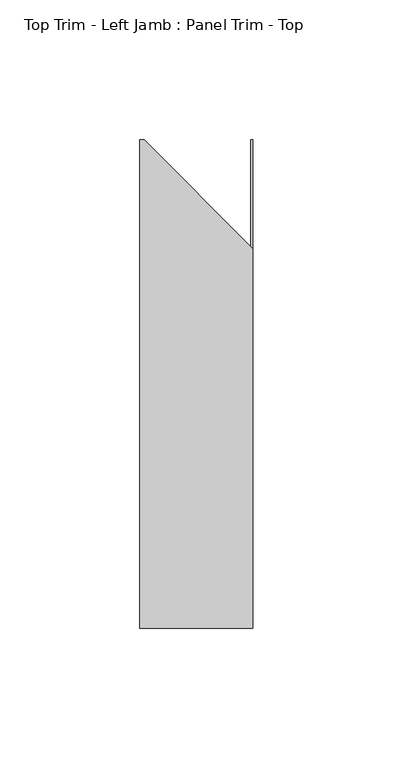
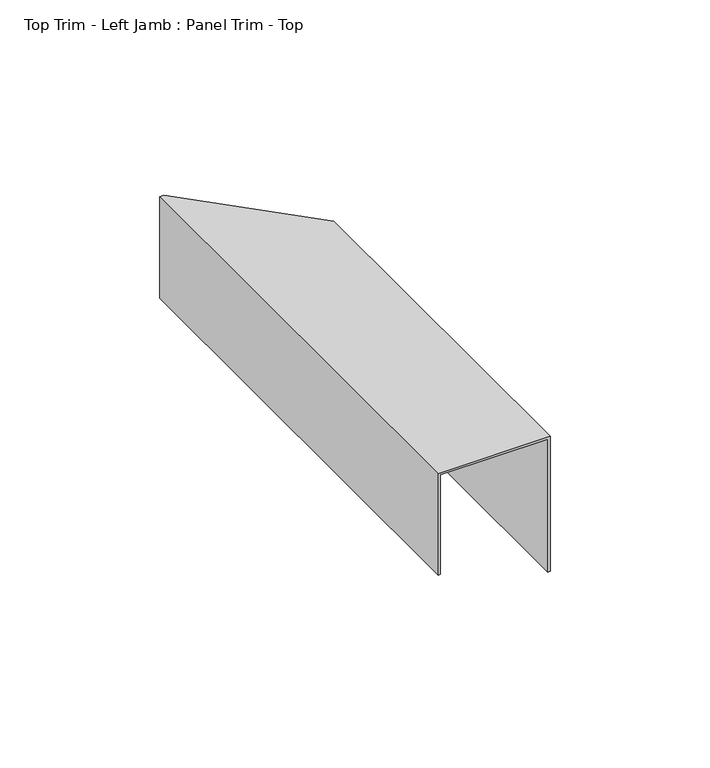
"""IFC4 building model written with IfcOpenShell, lengths in millimetres: proxy geometry, Top Trim - Left Jamb : Panel Trim - Top."""

import ifcopenshell
import ifcopenshell.guid

model = None  # the IFC model being written
_history = None  # IfcOwnerHistory: only IFC2X3 demands one
_inside = {}  # id of a spatial element -> (the spatial element, [elements in it])
_under = {}  # id of a project, library or spatial element -> (it, [spatial elements below it])
_declared = {}  # id of a project -> (the project, [libraries it declares])
_typed = {}  # id of a type object -> (the type object, [elements of that type])
_made_of = {}  # id of a material, layer set ... -> (it, [elements and type objects made of it])


def new_model(schema):
    """Start an empty IFC model of exactly this schema.

    Asked for "IFC4X3", IfcOpenShell would pick the latest addendum, in which some entities
    have other attributes; the version numbers below select the first issue.
    IFC2X3 requires an IfcOwnerHistory on every rooted entity: one is made here for all.
    """
    global model, _history
    if schema == "IFC4X3":
        model = ifcopenshell.file(schema_version=(4, 3, 0, 0))
    else:
        model = ifcopenshell.file(schema=schema)
    _inside.clear()
    _under.clear()
    _declared.clear()
    _typed.clear()
    _made_of.clear()
    _history = None
    if model.schema == "IFC2X3":
        org = make("IfcOrganization", Name="unknown")
        user = make(
            "IfcPersonAndOrganization",
            ThePerson=make("IfcPerson", FamilyName="unknown"),
            TheOrganization=org,
        )
        app = make(
            "IfcApplication",
            ApplicationDeveloper=org,
            Version="unknown",
            ApplicationFullName="unknown",
            ApplicationIdentifier="unknown",
        )
        _history = make(
            "IfcOwnerHistory",
            OwningUser=user,
            OwningApplication=app,
            ChangeAction="ADDED",
            CreationDate=0,
        )
    return model


def make(cls, **values):
    """One entity of the class cls with the attributes given. An attribute that is None is left unset."""
    return model.create_entity(
        cls, **{name: value for name, value in values.items() if value is not None}
    )


def rooted(cls, **values):
    """An entity with a GlobalId (a new one), such as an element, a storey or a relation."""
    return make(cls, GlobalId=ifcopenshell.guid.new(), OwnerHistory=_history, **values)


def si_unit(unit_type, name, prefix=None):
    """IfcSIUnit, for example si_unit("LENGTHUNIT", "METRE", prefix="MILLI")."""
    return make("IfcSIUnit", UnitType=unit_type, Prefix=prefix, Name=name)


def assignment(units):
    """IfcUnitAssignment: the units of a project."""
    return None if units is None else make("IfcUnitAssignment", Units=units)


def point(xyz):
    """IfcCartesianPoint."""
    return None if xyz is None else make("IfcCartesianPoint", Coordinates=xyz)


def direction(xyz):
    """IfcDirection."""
    return None if xyz is None else make("IfcDirection", DirectionRatios=xyz)


def frame(location, z_axis=None, x_axis=None):
    """IfcAxis2Placement3D, a coordinate frame: its origin and axes. An axis left out is left unset."""
    return make(
        "IfcAxis2Placement3D",
        Location=point(location),
        Axis=direction(z_axis),
        RefDirection=direction(x_axis),
    )


def origin():
    """The frame at (0, 0, 0) with its axes left unset."""
    return frame((0.0, 0.0, 0.0))


def place(relative_to, where):
    """IfcLocalPlacement: puts the frame where relative to a parent placement (None: the world)."""
    return make(
        "IfcLocalPlacement", PlacementRelTo=relative_to, RelativePlacement=where
    )


def context(
    kind, dimensions, precision=None, world=None, true_north=None, identifier=None
):
    """IfcGeometricRepresentationContext, for example the 3D "Model" context."""
    return make(
        "IfcGeometricRepresentationContext",
        ContextIdentifier=identifier,
        ContextType=kind,
        CoordinateSpaceDimension=dimensions,
        Precision=precision,
        WorldCoordinateSystem=world,
        TrueNorth=true_north,
    )


def project(units=None, contexts=None):
    """IfcProject with its units and contexts."""
    return rooted(
        "IfcProject",
        Name="project",
        RepresentationContexts=contexts,
        UnitsInContext=assignment(units),
    )


def spatial(cls, under=None, at=None, **own):
    """A site, building, storey or space (cls), placed at a placement, below another one or the project."""
    s = rooted(cls, ObjectPlacement=at, **own)
    if under is not None:
        _under.setdefault(under.id(), (under, []))[1].append(s)
    return s


def faces_of(points, faces, orient=None, outer=None):
    """IfcFace entities. A face is a list of loops; a loop is a list of indices into points, from 0.

    orient and outer hold one flag for each loop. By default every Orientation is true, the
    first loop of a face is its IfcFaceOuterBound and the others are IfcFaceBound.
    """
    made = []
    for i, loops in enumerate(faces):
        bounds = []
        for j, loop in enumerate(loops):
            is_outer = j == 0 if outer is None else outer[i][j]
            bounds.append(
                make(
                    "IfcFaceOuterBound" if is_outer else "IfcFaceBound",
                    Bound=make("IfcPolyLoop", Polygon=[points[k] for k in loop]),
                    Orientation=True if orient is None else orient[i][j],
                )
            )
        made.append(make("IfcFace", Bounds=bounds))
    return made


def faceted_brep(points, faces, orient=None, outer=None, voids=None):
    """IfcFacetedBrep: a solid bounded by flat faces; with voids (closed shells), ...WithVoids."""
    shared = [point(p) for p in points]
    hull = make("IfcClosedShell", CfsFaces=faces_of(shared, faces, orient, outer))
    if voids is None:
        return make("IfcFacetedBrep", Outer=hull)
    return make(
        "IfcFacetedBrepWithVoids",
        Outer=hull,
        Voids=[
            make(cls, CfsFaces=faces_of(shared, fs, o, b)) for cls, fs, o, b in voids
        ],
    )


def shape(context_of_items, identifier, shape_type, items):
    """IfcShapeRepresentation: the items that make up one representation, for example the "Body"."""
    return make(
        "IfcShapeRepresentation",
        ContextOfItems=context_of_items,
        RepresentationIdentifier=identifier,
        RepresentationType=shape_type,
        Items=items,
    )


def source(mapping_origin, context_of_items, identifier, shape_type, items):
    """IfcRepresentationMap: a shape defined once, which mapped items show again and again."""
    return make(
        "IfcRepresentationMap",
        MappingOrigin=mapping_origin,
        MappedRepresentation=shape(context_of_items, identifier, shape_type, items),
    )


def transform(
    local_origin,
    x_axis=None,
    y_axis=None,
    z_axis=None,
    scale=None,
    scale2=None,
    scale3=None,
    uniform=True,
):
    """IfcCartesianTransformationOperator3D, or its non-uniform kind. x_axis, y_axis, z_axis: its Axis1, 2, 3."""
    if uniform:
        return make(
            "IfcCartesianTransformationOperator3D",
            Axis1=direction(x_axis),
            Axis2=direction(y_axis),
            LocalOrigin=point(local_origin),
            Scale=scale,
            Axis3=direction(z_axis),
        )
    return make(
        "IfcCartesianTransformationOperator3DnonUniform",
        Axis1=direction(x_axis),
        Axis2=direction(y_axis),
        LocalOrigin=point(local_origin),
        Scale=scale,
        Axis3=direction(z_axis),
        Scale2=scale2,
        Scale3=scale3,
    )


def mapped(mapping_source, mapping_target):
    """IfcMappedItem: shows the shape of a source again, moved by a transform."""
    return make(
        "IfcMappedItem", MappingSource=mapping_source, MappingTarget=mapping_target
    )


def made_of(thing, what):
    """Note that an element or type object is made of a material, layer set ...; save() writes the relation."""
    if what is not None:
        _made_of.setdefault(what.id(), (what, []))[1].append(thing)
    return thing


def element(
    cls,
    number,
    at=None,
    inside=None,
    cuts=None,
    type_object=None,
    material=None,
    context=None,
    identifier="Body",
    shape_type=None,
    held_by="IfcProductDefinitionShape",
    body=None,
    shapes=None,
    **own,
):
    """One element of the class cls, such as IfcWall. Its Tag is "e" and its number.

    at: its placement. inside: the storey or other place that contains it. cuts: it is an
    opening in that element (IfcRelVoidsElement). A single representation is given by context,
    identifier, shape_type and body (its items); several are given by shapes. held_by: the class
    of the entity that holds the representations. save() writes the other relations.
    """
    e = rooted(cls, Tag="e%d" % number, ObjectPlacement=at, **own)
    if body is not None:
        shapes = [shape(context, identifier, shape_type, body)]
    if shapes is not None:
        e.Representation = make(held_by, Representations=shapes)
    if inside is not None:
        _inside.setdefault(inside.id(), (inside, []))[1].append(e)
    if cuts is not None:
        rooted(
            "IfcRelVoidsElement", RelatingBuildingElement=cuts, RelatedOpeningElement=e
        )
    if type_object is not None:
        _typed.setdefault(type_object.id(), (type_object, []))[1].append(e)
    return made_of(e, material)


def aggregate(whole, parts):
    """IfcRelAggregates: a whole, such as a stair, and the parts it consists of."""
    return rooted("IfcRelAggregates", RelatingObject=whole, RelatedObjects=parts)


def save(model, path):
    """Write the relations noted so far, then the file.

    IfcRelAggregates (storeys below a building ...), IfcRelContainedInSpatialStructure (elements
    in a storey), IfcRelDefinesByType, IfcRelAssociatesMaterial and IfcRelDeclares: one each for
    every whole, place, type object, material and project.
    """
    for whole, parts in _under.values():
        aggregate(whole, parts)
    for where, things in _inside.values():
        rooted(
            "IfcRelContainedInSpatialStructure",
            RelatedElements=things,
            RelatingStructure=where,
        )
    for kind, things in _typed.values():
        rooted("IfcRelDefinesByType", RelatedObjects=things, RelatingType=kind)
    for what, things in _made_of.values():
        rooted("IfcRelAssociatesMaterial", RelatedObjects=things, RelatingMaterial=what)
    for by, libraries in _declared.values():
        rooted("IfcRelDeclares", RelatingContext=by, RelatedDefinitions=libraries)
    model.write(path)


def top_trim_left_jamb_panel_trim_top_cc1ac03c(model_context):
    return source(origin(), model_context, "Body", "Brep", [
        faceted_brep([(587327.0060739, -531601.1163841, 2439.9875), (587327.0060739, -531601.1163841, 2401.8875), (587326.2186739, -531601.1163841, 2401.8875), (587326.2186739, -531601.1163841, 2440.78125), (587327.7847411, -531601.1163841, 2440.78125), (587327.7847411, -531601.1163841, 2439.9875), (587366.6808739, -531601.1163841, 2389.1875), (587365.8934739, -531601.1163841, 2389.1875), (587365.8934739, -531601.1163841, 2413.0), (587366.6808739, -531601.1163841, 2413.0), (587327.0060739, -531775.7413841, 2439.9875), (587365.8934739, -531775.7413841, 2439.9875), (587365.8934739, -531775.7413841, 2389.1875), (587366.6808739, -531775.7413841, 2389.1875), (587366.6808739, -531775.7413841, 2440.78125), (587326.2186739, -531775.7413841, 2440.78125), (587326.2186739, -531775.7413841, 2401.8875), (587327.0060739, -531775.7413841, 2401.8875), (587366.6808739, -531640.0125169, 2440.78125), (587366.6808739, -531640.0125169, 2413.0), (587365.8934739, -531639.2251169, 2439.9875), (587365.8934739, -531639.2251169, 2413.0)], [[[0, 1, 2, 3, 4, 5]], [[6, 7, 8, 9]], [[10, 11, 12, 13, 14, 15, 16, 17]], [[1, 0, 10, 17]], [[2, 1, 17, 16]], [[3, 2, 16, 15]], [[15, 14, 18, 4, 3]], [[14, 13, 6, 9, 19, 18]], [[7, 6, 13, 12]], [[12, 11, 20, 21, 8, 7]], [[11, 10, 0, 5, 20]], [[21, 19, 9, 8]], [[19, 21, 20, 5, 4, 18]]]),
    ])


if __name__ == "__main__":
    model = new_model("IFC4")
    model_context = context("Model", 3, world=origin())
    ifc_project = project(units=[si_unit("LENGTHUNIT", "METRE", prefix="MILLI")], contexts=[model_context])
    site = spatial("IfcSite", under=ifc_project)
    building = spatial("IfcBuilding", under=site)
    placement = place(None, origin())
    top_trim_left_jamb_panel_trim_top_shape = top_trim_left_jamb_panel_trim_top_cc1ac03c(model_context)
    element("IfcBuildingElementProxy", 1, Name="Top Trim - Left Jamb : Panel Trim - Top", ObjectType="Top Trim - Left Jamb : Panel Trim - Top", at=placement, inside=building, context=model_context, shape_type="MappedRepresentation", body=[
        mapped(top_trim_left_jamb_panel_trim_top_shape, transform((0.0, 0.0, 0.0), x_axis=(1.0, 0.0, 0.0), y_axis=(0.0, 1.0, 0.0), z_axis=(0.0, 0.0, 1.0))),
    ])
    save(model, "model.ifc")

# Revit data of these elements
# Element 1 (IfcBuildingElementProxy, "Top Trim - Left Jamb : Panel Trim - Top")
#   Materials on its faces: "EDGE TRIM BY MTL PANEL MFR."
# Materials
#   "EDGE TRIM BY MTL PANEL MFR.": class "Generic", colour RGB 239 242 240, transparency 0, Cost = 0
